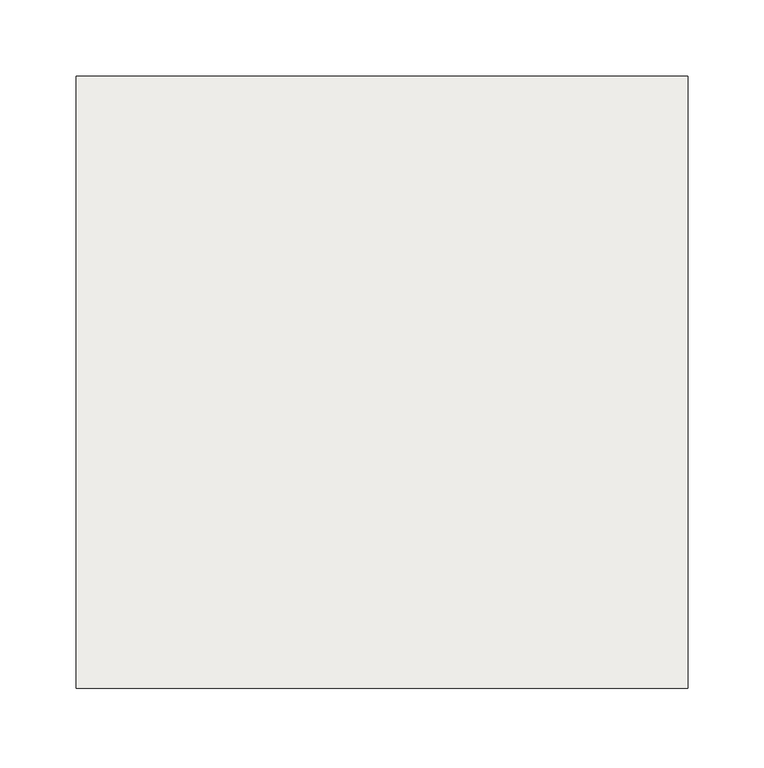
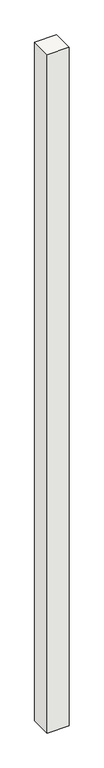
"""IFC4 building model written with IfcOpenShell, lengths in millimetres: footing geometry, NLRS_17_SFO_TLB_funderingspaal geheid beton prefab-AV-MMBPC_gen_rsf : heipaal beton prefab_gen__bxh 400x400."""

from ifc_helpers import new_model, si_unit, frame, origin, place, context, project, spatial, polyline, outline, extrude, source, transform, mapped, element, save


def footing_443494b9(model_context):
    return source(origin(), model_context, "Body", "SweptSolid", [
        extrude(outline(polyline([(200.0, -200.0), (-200.0, -200.0), (-200.0, 200.0), (200.0, 200.0), (200.0, -200.0)])), frame((0.0, 0.0, -20000.0), z_axis=(0.0, 0.0, 1.0), x_axis=(1.0, 0.0, 0.0)), (0.0, 0.0, 1.0), 13220.0),
    ])


if __name__ == "__main__":
    model = new_model("IFC4")
    model_context = context("Model", 3, world=origin())
    ifc_project = project(units=[si_unit("LENGTHUNIT", "METRE", prefix="MILLI")], contexts=[model_context])
    site = spatial("IfcSite", under=ifc_project)
    building = spatial("IfcBuilding", under=site)
    placement = place(None, origin())
    footing_shape = footing_443494b9(model_context)
    element("IfcFooting", 1, ObjectType="NLRS_17_SFO_TLB_funderingspaal geheid beton prefab-AV-MMBPC_gen_rsf : heipaal beton prefab_gen__bxh 400x400", at=placement, inside=building, context=model_context, shape_type="MappedRepresentation", body=[
        mapped(footing_shape, transform((0.0, 0.0, 0.0), x_axis=(1.0, 0.0, 0.0), y_axis=(0.0, 1.0, 0.0), z_axis=(0.0, 0.0, 1.0))),
    ])
    save(model, "model.ifc")

# Revit data of these elements
# Type "NLRS_17_SFO_TLB_funderingspaal geheid beton prefab-AV-MMBPC_gen_rsf : heipaal beton prefab_gen__bxh 400x400"
#   IfcExportAs = "IfcPile"
#   Type Comments = "prefab heipaal 400x400"
#   Model = " "
#   Manufacturer = " "
#   Description = "prefab heipaal 400x400"
#   Assembly Code = "17.21"
#   Width = 400 mm
#   Slanted Angle [instance default] = 0.00°
#   NLRS_S_draagvermogen_trek [instance default] = 0.00 kN
#   NLRS_S_draagvermogen_druk [instance default] = 0.00 kN
#   NLRS_C_lengte [instance default] = 1660 mm
#   NLRS_C_hoogte = 400 mm
#   NLRS_C_breedte = 400 mm
#   Height [instance default] = 1660 mm
#   Length [instance default] = 1660 mm
#   Angle [instance default] = 0.00°
#   Slanted [instance default] = 0
#   Structural Material = NLRS_f2_beton prefab_gen_rsf
#   Keynote = ""
# Element 1 (IfcFooting, "NLRS_17_SFO_TLB_funderingspaal geheid beton prefab-AV-MMBPC_gen_rsf : heipaal beton prefab_gen__bxh 400x400")
#   NLRS_C_lengte = 13220 mm
#   Height = 13220 mm
#   Length = 13220 mm
#   Materials on its faces: "NLRS_f2_beton prefab_gen_rsf"
# Materials
#   "NLRS_f2_beton prefab_gen_rsf": class "F - Niet gebakken kunststeen", colour RGB 129 133 118, transparency 0, Keynote = "f2", Manufacturer = "Revit Standards Foundation", URL = "www.revitstandards.org", Description = "beton prefab", Cost = 0
